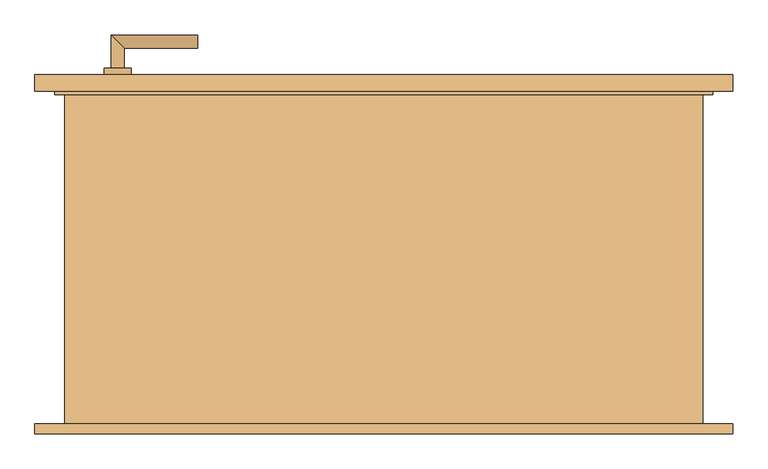
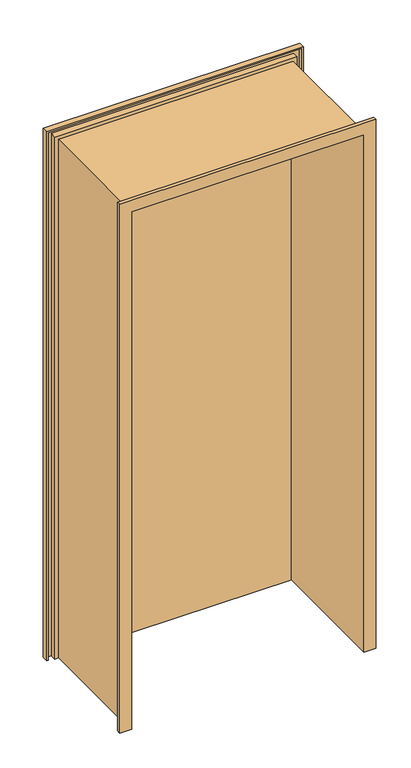
"""IFC4 building model written with IfcOpenShell, lengths in millimetres: door geometry, Drehflügel 1-flg - Variabel : Drehflügel 1-flg - Variabel."""

from ifc_helpers import new_model, si_unit, point, frame, frame_2d, origin, origin_with_axes, place, context, project, spatial, polyline, circle_curve, ellipse_curve, trimmed, segment, composite_curve, outline, extrude, faceted_brep, source, transform, mapped, element, save
from ifc_brep_helpers import plane_surface, cylinder_surface, advanced_brep


def door_07b48b99(model_context):
    return source(origin(), model_context, "Body", "SolidModel", [
        advanced_brep(
        [(-410.0, 239.4346141, 900.0), (-390.0, 239.4346141, 900.0), (-410.0, 169.4346141, 900.0), (-390.0, 189.4346141, 900.0), (-280.0, 169.4346141, 900.0), (-280.0, 189.4346141, 900.0)],
        [
            (0, 1, circle_curve(frame((-400.0, 239.4346141, 900.0), z_axis=(0.0, 1.0, 0.0), x_axis=(1.0, 0.0, 0.0)), 10.0)),
            (1, 0, circle_curve(frame((-400.0, 239.4346141, 900.0), z_axis=(0.0, 1.0, 0.0), x_axis=(1.0, 0.0, 0.0)), 10.0)),
            (0, 2),
            (2, 3, ellipse_curve(frame((-400.0, 179.4346141, 900.0), z_axis=(-0.7071067811865385, 0.7071067811865565, 0.0), x_axis=(0.7071067811865563, 0.7071067811865386, 0.0)), 14.1421356, 10.0)),
            (3, 1),
            (3, 2, ellipse_curve(frame((-400.0, 179.4346141, 900.0), z_axis=(-0.7071067811865385, 0.7071067811865565, 0.0), x_axis=(0.7071067811865563, 0.7071067811865386, 0.0)), 14.1421356, 10.0)),
            (4, 5, circle_curve(frame((-280.0, 179.4346141, 900.0), z_axis=(1.0, 0.0, 0.0), x_axis=(0.0, 1.0, 0.0)), 10.0)),
            (5, 4, circle_curve(frame((-280.0, 179.4346141, 900.0), z_axis=(1.0, 0.0, 0.0), x_axis=(0.0, 1.0, 0.0)), 10.0)),
            (2, 4),
            (5, 3),
        ],
        [
            plane_surface(frame((-400.0, 239.4346141, -387.7526403), z_axis=(0.0, 1.0, 0.0), x_axis=(0.0, 0.0, 1.0))),
            cylinder_surface(frame((-400.0, 239.4346141, 900.0), z_axis=(0.0, 1.0, 0.0), x_axis=(1.0, 0.0, 0.0)), 10.0),
            plane_surface(frame((-280.0, 179.4346141, -387.7526403), z_axis=(1.0, 0.0, 0.0), x_axis=(0.0, 0.0, 1.0))),
            cylinder_surface(frame((-400.0, 179.4346141, 900.0), z_axis=(-1.0, 0.0, 0.0), x_axis=(0.0, 1.0, 0.0)), 10.0),
        ],
        [
            (0, [[1, 2]]),
            (1, [[-1, 3, 4, 5]]),
            (1, [[-2, -5, 6, -3]]),
            (2, [[7, 8]]),
            (3, [[-4, 9, -8, 10]]),
            (3, [[-6, -10, -7, -9]]),
        ],
    ),
        advanced_brep(
        [(-390.0, 299.4346141, 900.0), (-410.0, 299.4346141, 900.0), (-390.0, 329.4346141, 900.0), (-410.0, 349.4346141, 900.0), (-280.0, 329.4346141, 900.0), (-280.0, 349.4346141, 900.0)],
        [
            (0, 1, circle_curve(frame((-400.0, 299.4346141, 900.0), z_axis=(0.0, -1.0, 0.0), x_axis=(-1.0, 0.0, 0.0)), 10.0)),
            (1, 0, circle_curve(frame((-400.0, 299.4346141, 900.0), z_axis=(0.0, -1.0, 0.0), x_axis=(-1.0, 0.0, 0.0)), 10.0)),
            (0, 2),
            (2, 3, ellipse_curve(frame((-400.0, 339.4346141, 900.0), z_axis=(-0.7071067811865475, -0.7071067811865475, 0.0), x_axis=(0.7071067811865474, -0.7071067811865476, 0.0)), 14.1421356, 10.0)),
            (3, 1),
            (3, 2, ellipse_curve(frame((-400.0, 339.4346141, 900.0), z_axis=(-0.7071067811865475, -0.7071067811865475, 0.0), x_axis=(0.7071067811865474, -0.7071067811865476, 0.0)), 14.1421356, 10.0)),
            (4, 5, circle_curve(frame((-280.0, 339.4346141, 900.0), z_axis=(1.0, 0.0, 0.0), x_axis=(0.0, 1.0, 0.0)), 10.0)),
            (5, 4, circle_curve(frame((-280.0, 339.4346141, 900.0), z_axis=(1.0, 0.0, 0.0), x_axis=(0.0, 1.0, 0.0)), 10.0)),
            (2, 4),
            (5, 3),
        ],
        [
            plane_surface(frame((-400.0, 299.4346141, -387.7526403), z_axis=(0.0, -1.0, 0.0), x_axis=(0.0, 0.0, 1.0))),
            cylinder_surface(frame((-400.0, 299.4346141, 900.0), z_axis=(0.0, -1.0, 0.0), x_axis=(-1.0, 0.0, 0.0)), 10.0),
            plane_surface(frame((-280.0, 339.4346141, -387.7526403), z_axis=(1.0, 0.0, 0.0), x_axis=(0.0, 0.0, 1.0))),
            cylinder_surface(frame((-400.0, 339.4346141, 900.0), z_axis=(-1.0, 0.0, 0.0), x_axis=(0.0, 1.0, 0.0)), 10.0),
        ],
        [
            (0, [[1, 2]]),
            (1, [[-1, 3, 4, 5]]),
            (1, [[-2, -5, 6, -3]]),
            (2, [[7, 8]]),
            (3, [[-4, 9, -8, 10]]),
            (3, [[-6, -10, -7, -9]]),
        ],
    ),
        extrude(outline(composite_curve([segment(trimmed(circle_curve(frame_2d((900.0, -400.0)), 20.0), [point((900.0, -420.0))], [point((900.0, -380.0))], False, "CARTESIAN"), True, "CONTINUOUS"), segment(trimmed(circle_curve(frame_2d((900.0, -400.0)), 20.0), [point((900.0, -380.0))], [point((900.0, -420.0))], False, "CARTESIAN"), True, "CONTINUOUS")], self_intersect=False)), frame((0.0, 229.4346141, 0.0), z_axis=(0.0, 1.0, 0.0), x_axis=(0.0, 0.0, 1.0)), (0.0, 0.0, 1.0), 10.0),
        extrude(outline(composite_curve([segment(trimmed(circle_curve(frame_2d((900.0, -400.0)), 20.0), [point((900.0, -420.0))], [point((900.0, -380.0))], False, "CARTESIAN"), True, "CONTINUOUS"), segment(trimmed(circle_curve(frame_2d((900.0, -400.0)), 20.0), [point((900.0, -380.0))], [point((900.0, -420.0))], False, "CARTESIAN"), True, "CONTINUOUS")], self_intersect=False)), frame((0.0, 289.4346141, 0.0), z_axis=(0.0, 1.0, 0.0), x_axis=(0.0, 0.0, 1.0)), (0.0, 0.0, 1.0), 10.0),
        extrude(outline(polyline([(490.0, 264.4346141), (-490.0, 264.4346141), (-490.0, 289.4346141), (490.0, 289.4346141), (490.0, 264.4346141)])), origin_with_axes(), (0.0, 0.0, 1.0), 2250.0),
        faceted_brep([(524.4603207, -250.5653859, 0.0), (475.0, -250.5653859, 0.0), (475.0, 264.4346141, 0.0), (490.0, 264.4346141, 0.0), (490.0, 289.4346141, 0.0), (524.4603207, 289.4346141, 0.0), (524.4603207, 264.4346141, 0.0), (519.4603207, 264.4346141, 0.0), (519.4603207, 284.4346141, 0.0), (495.0, 284.4346141, 0.0), (495.0, 259.4346141, 0.0), (480.0, 259.4346141, 0.0), (480.0, -245.5653859, 0.0), (519.4603207, -245.5653859, 0.0), (519.4603207, -235.5653859, 0.0), (524.4603207, -235.5653859, 0.0), (524.4603207, -250.5653859, 2284.4603207), (-524.4603207, -250.5653859, 2284.4603207), (-524.4603207, -250.5653859, 0.0), (-475.0, -250.5653859, 0.0), (-475.0, -250.5653859, 2235.0), (475.0, -250.5653859, 2235.0), (475.0, 264.4346141, 2235.0), (-475.0, 264.4346141, 2235.0), (-475.0, 264.4346141, 0.0), (-490.0, 264.4346141, 0.0), (-490.0, 264.4346141, 2250.0), (490.0, 264.4346141, 2250.0), (490.0, 289.4346141, 2250.0), (-490.0, 289.4346141, 2250.0), (-490.0, 289.4346141, 0.0), (-524.4603207, 289.4346141, 0.0), (-524.4603207, 289.4346141, 2284.4603207), (524.4603207, 289.4346141, 2284.4603207), (524.4603207, 264.4346141, 2284.4603207), (-524.4603207, 264.4346141, 2284.4603207), (-524.4603207, 264.4346141, 0.0), (-519.4603207, 264.4346141, 0.0), (-519.4603207, 264.4346141, 2279.4603207), (519.4603207, 264.4346141, 2279.4603207), (519.4603207, 284.4346141, 2279.4603207), (-519.4603207, 284.4346141, 2279.4603207), (-519.4603207, 284.4346141, 0.0), (-495.0, 284.4346141, 0.0), (-495.0, 284.4346141, 2255.0), (495.0, 284.4346141, 2255.0), (495.0, 259.4346141, 2255.0), (-495.0, 259.4346141, 2255.0), (-495.0, 259.4346141, 0.0), (-480.0, 259.4346141, 0.0), (-480.0, 259.4346141, 2240.0), (480.0, 259.4346141, 2240.0), (480.0, -245.5653859, 2240.0), (-480.0, -245.5653859, 2240.0), (-480.0, -245.5653859, 0.0), (-519.4603207, -245.5653859, 0.0), (-519.4603207, -245.5653859, 2279.4603207), (519.4603207, -245.5653859, 2279.4603207), (519.4603207, -235.5653859, 2279.4603207), (-519.4603207, -235.5653859, 2279.4603207), (-519.4603207, -235.5653859, 0.0), (-524.4603207, -235.5653859, 0.0), (-524.4603207, -235.5653859, 2284.4603207), (524.4603207, -235.5653859, 2284.4603207)], [[[0, 1, 2, 3, 4, 5, 6, 7, 8, 9, 10, 11, 12, 13, 14, 15]], [[1, 0, 16, 17, 18, 19, 20, 21]], [[2, 1, 21, 22]], [[3, 2, 22, 23, 24, 25, 26, 27]], [[4, 3, 27, 28]], [[5, 4, 28, 29, 30, 31, 32, 33]], [[6, 5, 33, 34]], [[7, 6, 34, 35, 36, 37, 38, 39]], [[8, 7, 39, 40]], [[9, 8, 40, 41, 42, 43, 44, 45]], [[10, 9, 45, 46]], [[11, 10, 46, 47, 48, 49, 50, 51]], [[12, 11, 51, 52]], [[13, 12, 52, 53, 54, 55, 56, 57]], [[14, 13, 57, 58]], [[15, 14, 58, 59, 60, 61, 62, 63]], [[0, 15, 63, 16]], [[17, 62, 61, 18]], [[18, 61, 60, 55, 54, 49, 48, 43, 42, 37, 36, 31, 30, 25, 24, 19]], [[23, 20, 19, 24]], [[29, 26, 25, 30]], [[35, 32, 31, 36]], [[41, 38, 37, 42]], [[47, 44, 43, 48]], [[53, 50, 49, 54]], [[59, 56, 55, 60]], [[22, 21, 20, 23]], [[28, 27, 26, 29]], [[34, 33, 32, 35]], [[40, 39, 38, 41]], [[46, 45, 44, 47]], [[52, 51, 50, 53]], [[58, 57, 56, 59]], [[16, 63, 62, 17]]]),
    ])


if __name__ == "__main__":
    model = new_model("IFC4")
    model_context = context("Model", 3, world=origin())
    ifc_project = project(units=[si_unit("LENGTHUNIT", "METRE", prefix="MILLI")], contexts=[model_context])
    site = spatial("IfcSite", under=ifc_project)
    building = spatial("IfcBuilding", under=site)
    placement = place(None, origin())
    door_shape = door_07b48b99(model_context)
    element("IfcDoor", 1, ObjectType="Drehflügel 1-flg - Variabel : Drehflügel 1-flg - Variabel", at=placement, inside=building, context=model_context, shape_type="MappedRepresentation", body=[
        mapped(door_shape, transform((0.0, 0.0, 0.0), x_axis=(1.0, 0.0, 0.0), y_axis=(0.0, 1.0, 0.0), z_axis=(0.0, 0.0, 1.0))),
    ])
    save(model, "model.ifc")

# Revit data of these elements
# Type "Drehflügel 1-flg - Variabel : Drehflügel 1-flg - Variabel"
#   Construction Type Id = "MDOOR"
#   Type Mark = "15"
#   Operation = "SingleSwingRight"
#   Keynote = "16.03"
#   Analytic Construction = "Metall"
#   Thermal Resistance (R) = 0.270117 (m²·K)/W
#   Heat Transfer Coefficient (U) = 3.7021 W/(m²·K)
#   Rough Width [instance default] = 1.000 m
#   Rough Height [instance default] = 2.360 m
#   Höhe Türgriff [instance default] = 0.900 m
#   Height [instance default] = 2.260 m
#   Fußbodenaufbau [instance default] = 0.100 m
#   Width [instance default] = 1.000 m
#   Sichtbarkeit Sturzlinien [instance default] = yes
#   Türgriff auswählen [instance default] = element 217699
#   Türgriff [instance default] = none
#   Türflügel [instance default] = none
#   Rahmen/Pfosten [instance default] = Metall - Lackiert - Grau
#   Visual Light Transmittance = 0
#   Solar Heat Gain Coefficient = 0
#   Function = (empty or 0)
#   Wall Closure = (empty or 0)
# Element 1 (IfcDoor, "Drehflügel 1-flg - Variabel : Drehflügel 1-flg - Variabel")
#   Rough Height = 2.260 m
#   Fußbodenaufbau = 0.000 m
#   Materials on its faces: "Metall - Lackiert - Grau", "Metall - Chrom", "Holz - Birke"
# Materials
#   "Metall - Lackiert - Grau": class "Farbe 1", colour RGB 98 98 98, transparency 0, Cost = 0
#   "Metall - Chrom": class "Metall", colour RGB 247 247 247, transparency 0, Cost = 0
#   "Holz - Birke": class "Holz", colour RGB 213 164 103, transparency 0, Cost = 0
